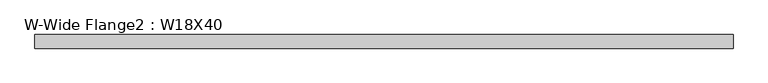
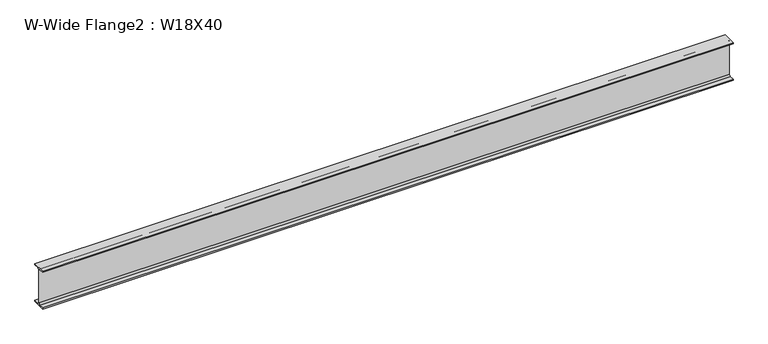
"""IFC4 building model written with IfcOpenShell, lengths in millimetres: beam geometry, W-Wide Flange2 : W18X40."""

from ifc_helpers import new_model, si_unit, point, frame, frame_2d, origin, place, context, project, spatial, polyline, circle_curve, trimmed, segment, composite_curve, outline, extrude, source, transform, mapped, element, save


def w_wide_flange2_w18x40_909044dc(model_context):
    return source(origin(), model_context, "Body", "SweptSolid", [
        extrude(outline(composite_curve([segment(polyline([(76.454, -213.995), (76.454, -227.33), (-76.454, -227.33), (-76.454, -213.995), (-20.828, -213.995)]), True, "CONTINUOUS"), segment(trimmed(circle_curve(frame_2d((-20.828, -197.1675)), 16.8275), [point((-20.828, -213.995))], [point((-4.0005, -197.1675))], True, "CARTESIAN"), True, "CONTINUOUS"), segment(polyline([(-4.0005, -197.1675), (-4.0005, 197.1675)]), True, "CONTINUOUS"), segment(trimmed(circle_curve(frame_2d((-20.828, 197.1675)), 16.8275), [point((-4.0005, 197.1675))], [point((-20.828, 213.995))], True, "CARTESIAN"), True, "CONTINUOUS"), segment(polyline([(-20.828, 213.995), (-76.454, 213.995), (-76.454, 227.33), (76.454, 227.33), (76.454, 213.995), (20.828, 213.995)]), True, "CONTINUOUS"), segment(trimmed(circle_curve(frame_2d((20.828, 197.1675)), 16.8275), [point((20.828, 213.995))], [point((4.0005, 197.1675))], True, "CARTESIAN"), True, "CONTINUOUS"), segment(polyline([(4.0005, 197.1675), (4.0005, -197.1675)]), True, "CONTINUOUS"), segment(trimmed(circle_curve(frame_2d((20.828, -197.1675)), 16.8275), [point((4.0005, -197.1675))], [point((20.828, -213.995))], True, "CARTESIAN"), True, "CONTINUOUS"), segment(polyline([(20.828, -213.995), (76.454, -213.995)]), True, "CONTINUOUS")], self_intersect=False)), frame((-3894.534375, 0.0, 0.0), z_axis=(1.0, 0.0, 0.0), x_axis=(0.0, 1.0, 0.0)), (0.0, 0.0, 1.0), 7851.378125),
    ])


if __name__ == "__main__":
    model = new_model("IFC4")
    model_context = context("Model", 3, world=origin())
    ifc_project = project(units=[si_unit("LENGTHUNIT", "METRE", prefix="MILLI")], contexts=[model_context])
    site = spatial("IfcSite", under=ifc_project)
    building = spatial("IfcBuilding", under=site)
    placement = place(None, origin())
    w_wide_flange2_w18x40_shape = w_wide_flange2_w18x40_909044dc(model_context)
    element("IfcBeam", 1, ObjectType="W-Wide Flange2 : W18X40", at=placement, inside=building, context=model_context, shape_type="MappedRepresentation", body=[
        mapped(w_wide_flange2_w18x40_shape, transform((0.0, 0.0, 0.0), x_axis=(1.0, 0.0, 0.0), y_axis=(0.0, 1.0, 0.0), z_axis=(0.0, 0.0, 1.0))),
    ])
    save(model, "model.ifc")

# Revit data of these elements
# Type "W-Wide Flange2 : W18X40"
#   Assembly Code = "B10"
#   W = 40
#   Length [instance default] = 5' - 0"
#   bf = 0' - 6.02"
#   d = 1' - 5.9"
#   k = 0' - 1 3/16"
#   k2 = 0' - 0.6625"
#   tf = 0' - 0.525"
#   tw = 0' - 0.315"
#   A = 0.0819444 SF
#   Structural Material [instance default] = Steel ASTM A992
# Element 1 (IfcBeam, "W-Wide Flange2 : W18X40")
#   Materials on its faces: "Steel ASTM A992"
# Materials
#   "Steel ASTM A992": class "Metal", colour RGB 199 199 199, transparency 0, Description = "Structural steel 50ksi", Cost = 0
